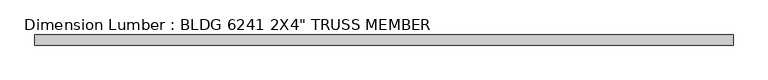
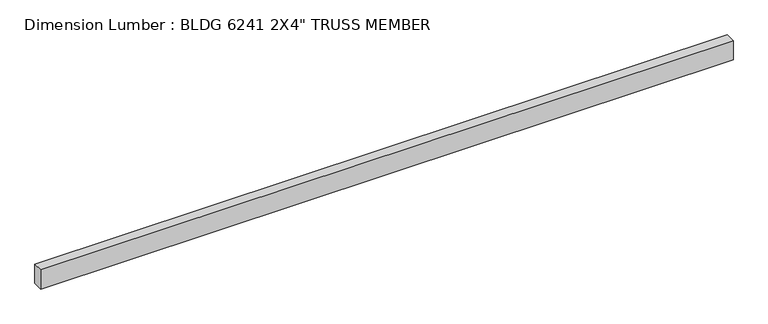
"""IFC4 building model written with IfcOpenShell, lengths in millimetres: beam geometry."""

from ifc_helpers import new_model, si_unit, frame, origin, place, context, project, spatial, polyline, outline, extrude, source, transform, mapped, element, save


def beam_717df711(model_context):
    return source(origin(), model_context, "Body", "SweptSolid", [
        extrude(outline(polyline([(1716.6789755, 25.4), (1716.6789755, -25.4), (-1777.9999994, -25.4), (-1777.9999994, 25.4), (1716.6789755, 25.4)])), frame((0.0, 0.0, -50.8), z_axis=(0.0, 0.0, 1.0), x_axis=(1.0, 0.0, 0.0)), (0.0, 0.0, 1.0), 101.6),
    ])


if __name__ == "__main__":
    model = new_model("IFC4")
    model_context = context("Model", 3, world=origin())
    ifc_project = project(units=[si_unit("LENGTHUNIT", "METRE", prefix="MILLI")], contexts=[model_context])
    site = spatial("IfcSite", under=ifc_project)
    building = spatial("IfcBuilding", under=site)
    placement = place(None, origin())
    beam_shape = beam_717df711(model_context)
    element("IfcBeam", 1, ObjectType="Dimension Lumber : BLDG 6241 2X4\" TRUSS MEMBER", at=placement, inside=building, context=model_context, shape_type="MappedRepresentation", body=[
        mapped(beam_shape, transform((0.0, 0.0, 0.0), x_axis=(1.0, 0.0, 0.0), y_axis=(0.0, 1.0, 0.0), z_axis=(0.0, 0.0, 1.0))),
    ])
    save(model, "model.ifc")

# Revit data of these elements
# Type "Dimension Lumber : BLDG 6241 2X4\" TRUSS MEMBER"
#   Assembly Code = "B10"
#   A = 0.273472 SF
#   Length [instance default] = 5' - 0"
#   b = 0' - 2"
#   d = 0' - 4"
#   Structural Material [instance default] = Softwood, Lumber
# Element 1 (IfcBeam, "Dimension Lumber : BLDG 6241 2X4\" TRUSS MEMBER")
#   Materials on its faces: "Softwood, Lumber"
# Materials
#   "Softwood, Lumber": class "Wood", colour RGB 223 192 134, transparency 0, Description = "Pinus Echinata", Cost = 0
